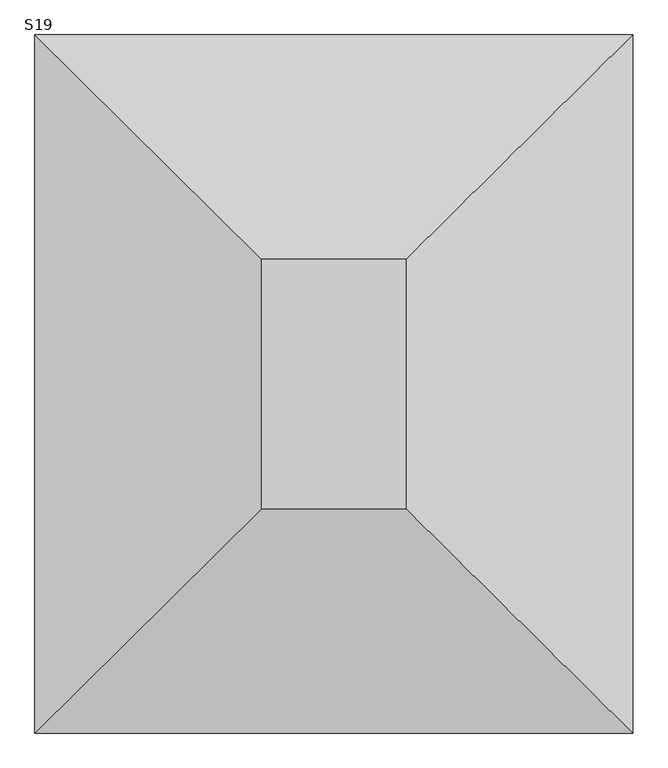
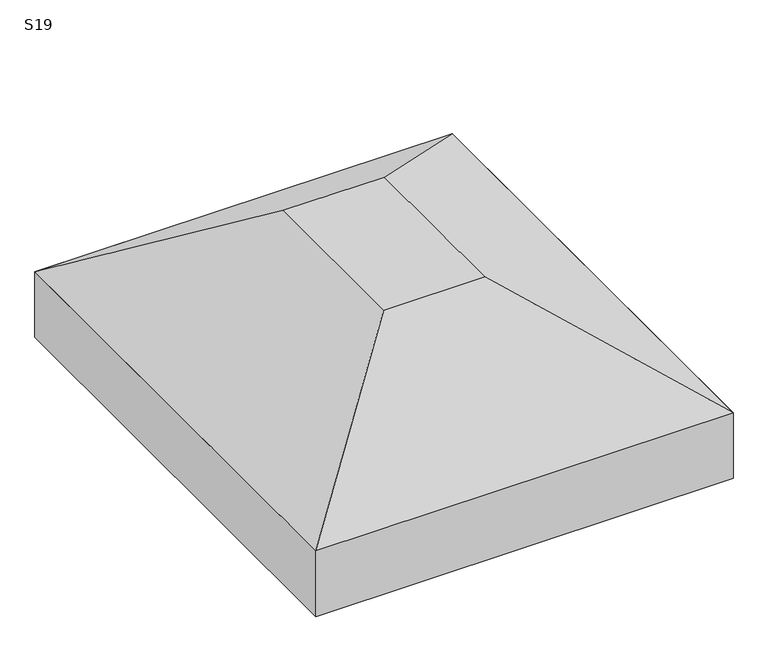
"""IFC4 building model written with IfcOpenShell, lengths in millimetres: fastener geometry, TQS - Sapata : S19."""

import ifcopenshell
import ifcopenshell.guid

model = None  # the IFC model being written
_history = None  # IfcOwnerHistory: only IFC2X3 demands one
_inside = {}  # id of a spatial element -> (the spatial element, [elements in it])
_under = {}  # id of a project, library or spatial element -> (it, [spatial elements below it])
_declared = {}  # id of a project -> (the project, [libraries it declares])
_typed = {}  # id of a type object -> (the type object, [elements of that type])
_made_of = {}  # id of a material, layer set ... -> (it, [elements and type objects made of it])


def new_model(schema):
    """Start an empty IFC model of exactly this schema.

    Asked for "IFC4X3", IfcOpenShell would pick the latest addendum, in which some entities
    have other attributes; the version numbers below select the first issue.
    IFC2X3 requires an IfcOwnerHistory on every rooted entity: one is made here for all.
    """
    global model, _history
    if schema == "IFC4X3":
        model = ifcopenshell.file(schema_version=(4, 3, 0, 0))
    else:
        model = ifcopenshell.file(schema=schema)
    _inside.clear()
    _under.clear()
    _declared.clear()
    _typed.clear()
    _made_of.clear()
    _history = None
    if model.schema == "IFC2X3":
        org = make("IfcOrganization", Name="unknown")
        user = make(
            "IfcPersonAndOrganization",
            ThePerson=make("IfcPerson", FamilyName="unknown"),
            TheOrganization=org,
        )
        app = make(
            "IfcApplication",
            ApplicationDeveloper=org,
            Version="unknown",
            ApplicationFullName="unknown",
            ApplicationIdentifier="unknown",
        )
        _history = make(
            "IfcOwnerHistory",
            OwningUser=user,
            OwningApplication=app,
            ChangeAction="ADDED",
            CreationDate=0,
        )
    return model


def make(cls, **values):
    """One entity of the class cls with the attributes given. An attribute that is None is left unset."""
    return model.create_entity(
        cls, **{name: value for name, value in values.items() if value is not None}
    )


def rooted(cls, **values):
    """An entity with a GlobalId (a new one), such as an element, a storey or a relation."""
    return make(cls, GlobalId=ifcopenshell.guid.new(), OwnerHistory=_history, **values)


def si_unit(unit_type, name, prefix=None):
    """IfcSIUnit, for example si_unit("LENGTHUNIT", "METRE", prefix="MILLI")."""
    return make("IfcSIUnit", UnitType=unit_type, Prefix=prefix, Name=name)


def assignment(units):
    """IfcUnitAssignment: the units of a project."""
    return None if units is None else make("IfcUnitAssignment", Units=units)


def point(xyz):
    """IfcCartesianPoint."""
    return None if xyz is None else make("IfcCartesianPoint", Coordinates=xyz)


def direction(xyz):
    """IfcDirection."""
    return None if xyz is None else make("IfcDirection", DirectionRatios=xyz)


def frame(location, z_axis=None, x_axis=None):
    """IfcAxis2Placement3D, a coordinate frame: its origin and axes. An axis left out is left unset."""
    return make(
        "IfcAxis2Placement3D",
        Location=point(location),
        Axis=direction(z_axis),
        RefDirection=direction(x_axis),
    )


def origin():
    """The frame at (0, 0, 0) with its axes left unset."""
    return frame((0.0, 0.0, 0.0))


def place(relative_to, where):
    """IfcLocalPlacement: puts the frame where relative to a parent placement (None: the world)."""
    return make(
        "IfcLocalPlacement", PlacementRelTo=relative_to, RelativePlacement=where
    )


def context(
    kind, dimensions, precision=None, world=None, true_north=None, identifier=None
):
    """IfcGeometricRepresentationContext, for example the 3D "Model" context."""
    return make(
        "IfcGeometricRepresentationContext",
        ContextIdentifier=identifier,
        ContextType=kind,
        CoordinateSpaceDimension=dimensions,
        Precision=precision,
        WorldCoordinateSystem=world,
        TrueNorth=true_north,
    )


def project(units=None, contexts=None):
    """IfcProject with its units and contexts."""
    return rooted(
        "IfcProject",
        Name="project",
        RepresentationContexts=contexts,
        UnitsInContext=assignment(units),
    )


def spatial(cls, under=None, at=None, **own):
    """A site, building, storey or space (cls), placed at a placement, below another one or the project."""
    s = rooted(cls, ObjectPlacement=at, **own)
    if under is not None:
        _under.setdefault(under.id(), (under, []))[1].append(s)
    return s


def polyline(points):
    """IfcPolyline through the points."""
    return make("IfcPolyline", Points=[point(p) for p in points])


def outline(outer, holes=None, kind="AREA"):
    """IfcArbitraryClosedProfileDef: a profile drawn as a closed curve; with holes, ...WithVoids."""
    if holes is None:
        return make("IfcArbitraryClosedProfileDef", ProfileType=kind, OuterCurve=outer)
    return make(
        "IfcArbitraryProfileDefWithVoids",
        ProfileType=kind,
        OuterCurve=outer,
        InnerCurves=holes,
    )


def extrude(swept, where, along, depth):
    """IfcExtrudedAreaSolid: the profile swept, set in the frame where, extruded along a direction by depth."""
    return make(
        "IfcExtrudedAreaSolid",
        SweptArea=swept,
        Position=where,
        ExtrudedDirection=direction(along),
        Depth=depth,
    )


def faces_of(points, faces, orient=None, outer=None):
    """IfcFace entities. A face is a list of loops; a loop is a list of indices into points, from 0.

    orient and outer hold one flag for each loop. By default every Orientation is true, the
    first loop of a face is its IfcFaceOuterBound and the others are IfcFaceBound.
    """
    made = []
    for i, loops in enumerate(faces):
        bounds = []
        for j, loop in enumerate(loops):
            is_outer = j == 0 if outer is None else outer[i][j]
            bounds.append(
                make(
                    "IfcFaceOuterBound" if is_outer else "IfcFaceBound",
                    Bound=make("IfcPolyLoop", Polygon=[points[k] for k in loop]),
                    Orientation=True if orient is None else orient[i][j],
                )
            )
        made.append(make("IfcFace", Bounds=bounds))
    return made


def faceted_brep(points, faces, orient=None, outer=None, voids=None):
    """IfcFacetedBrep: a solid bounded by flat faces; with voids (closed shells), ...WithVoids."""
    shared = [point(p) for p in points]
    hull = make("IfcClosedShell", CfsFaces=faces_of(shared, faces, orient, outer))
    if voids is None:
        return make("IfcFacetedBrep", Outer=hull)
    return make(
        "IfcFacetedBrepWithVoids",
        Outer=hull,
        Voids=[
            make(cls, CfsFaces=faces_of(shared, fs, o, b)) for cls, fs, o, b in voids
        ],
    )


def shape(context_of_items, identifier, shape_type, items):
    """IfcShapeRepresentation: the items that make up one representation, for example the "Body"."""
    return make(
        "IfcShapeRepresentation",
        ContextOfItems=context_of_items,
        RepresentationIdentifier=identifier,
        RepresentationType=shape_type,
        Items=items,
    )


def source(mapping_origin, context_of_items, identifier, shape_type, items):
    """IfcRepresentationMap: a shape defined once, which mapped items show again and again."""
    return make(
        "IfcRepresentationMap",
        MappingOrigin=mapping_origin,
        MappedRepresentation=shape(context_of_items, identifier, shape_type, items),
    )


def transform(
    local_origin,
    x_axis=None,
    y_axis=None,
    z_axis=None,
    scale=None,
    scale2=None,
    scale3=None,
    uniform=True,
):
    """IfcCartesianTransformationOperator3D, or its non-uniform kind. x_axis, y_axis, z_axis: its Axis1, 2, 3."""
    if uniform:
        return make(
            "IfcCartesianTransformationOperator3D",
            Axis1=direction(x_axis),
            Axis2=direction(y_axis),
            LocalOrigin=point(local_origin),
            Scale=scale,
            Axis3=direction(z_axis),
        )
    return make(
        "IfcCartesianTransformationOperator3DnonUniform",
        Axis1=direction(x_axis),
        Axis2=direction(y_axis),
        LocalOrigin=point(local_origin),
        Scale=scale,
        Axis3=direction(z_axis),
        Scale2=scale2,
        Scale3=scale3,
    )


def mapped(mapping_source, mapping_target):
    """IfcMappedItem: shows the shape of a source again, moved by a transform."""
    return make(
        "IfcMappedItem", MappingSource=mapping_source, MappingTarget=mapping_target
    )


def made_of(thing, what):
    """Note that an element or type object is made of a material, layer set ...; save() writes the relation."""
    if what is not None:
        _made_of.setdefault(what.id(), (what, []))[1].append(thing)
    return thing


def element(
    cls,
    number,
    at=None,
    inside=None,
    cuts=None,
    type_object=None,
    material=None,
    context=None,
    identifier="Body",
    shape_type=None,
    held_by="IfcProductDefinitionShape",
    body=None,
    shapes=None,
    **own,
):
    """One element of the class cls, such as IfcWall. Its Tag is "e" and its number.

    at: its placement. inside: the storey or other place that contains it. cuts: it is an
    opening in that element (IfcRelVoidsElement). A single representation is given by context,
    identifier, shape_type and body (its items); several are given by shapes. held_by: the class
    of the entity that holds the representations. save() writes the other relations.
    """
    e = rooted(cls, Tag="e%d" % number, ObjectPlacement=at, **own)
    if body is not None:
        shapes = [shape(context, identifier, shape_type, body)]
    if shapes is not None:
        e.Representation = make(held_by, Representations=shapes)
    if inside is not None:
        _inside.setdefault(inside.id(), (inside, []))[1].append(e)
    if cuts is not None:
        rooted(
            "IfcRelVoidsElement", RelatingBuildingElement=cuts, RelatedOpeningElement=e
        )
    if type_object is not None:
        _typed.setdefault(type_object.id(), (type_object, []))[1].append(e)
    return made_of(e, material)


def aggregate(whole, parts):
    """IfcRelAggregates: a whole, such as a stair, and the parts it consists of."""
    return rooted("IfcRelAggregates", RelatingObject=whole, RelatedObjects=parts)


def save(model, path):
    """Write the relations noted so far, then the file.

    IfcRelAggregates (storeys below a building ...), IfcRelContainedInSpatialStructure (elements
    in a storey), IfcRelDefinesByType, IfcRelAssociatesMaterial and IfcRelDeclares: one each for
    every whole, place, type object, material and project.
    """
    for whole, parts in _under.values():
        aggregate(whole, parts)
    for where, things in _inside.values():
        rooted(
            "IfcRelContainedInSpatialStructure",
            RelatedElements=things,
            RelatingStructure=where,
        )
    for kind, things in _typed.values():
        rooted("IfcRelDefinesByType", RelatedObjects=things, RelatingType=kind)
    for what, things in _made_of.values():
        rooted("IfcRelAssociatesMaterial", RelatedObjects=things, RelatingMaterial=what)
    for by, libraries in _declared.values():
        rooted("IfcRelDeclares", RelatingContext=by, RelatedDefinitions=libraries)
    model.write(path)


def s19_c62a4a8b(model_context):
    return source(origin(), model_context, "Body", "SolidModel", [
        faceted_brep([(-55.0, 50.0, 0.0), (-345.0, 50.0, 0.0), (-345.0, -450.0, 0.0), (-55.0, -450.0, 0.0), (400.0, 500.0, -300.0), (400.0, -900.0, -300.0), (-800.0, -900.0, -300.0), (-800.0, 500.0, -300.0)], [[[0, 1, 2, 3]], [[4, 5, 6, 7]], [[4, 7, 1, 0]], [[7, 6, 2, 1]], [[6, 5, 3, 2]], [[5, 4, 0, 3]]]),
        extrude(outline(polyline([(400.0, 500.0), (400.0, -900.0), (-800.0, -900.0), (-800.0, 500.0), (400.0, 500.0)])), frame((0.0, 0.0, -500.0), z_axis=(0.0, 0.0, 1.0), x_axis=(1.0, 0.0, 0.0)), (0.0, 0.0, 1.0), 200.0),
    ])


if __name__ == "__main__":
    model = new_model("IFC4")
    model_context = context("Model", 3, world=origin())
    ifc_project = project(units=[si_unit("LENGTHUNIT", "METRE", prefix="MILLI")], contexts=[model_context])
    site = spatial("IfcSite", under=ifc_project)
    building = spatial("IfcBuilding", under=site)
    placement = place(None, origin())
    s19_shape = s19_c62a4a8b(model_context)
    element("IfcFastener", 1, ObjectType="TQS - Sapata : S19", at=placement, inside=building, context=model_context, shape_type="MappedRepresentation", body=[
        mapped(s19_shape, transform((0.0, 0.0, 0.0), x_axis=(1.0, 0.0, 0.0), y_axis=(0.0, 1.0, 0.0), z_axis=(0.0, 0.0, 1.0))),
    ])
    save(model, "model.ifc")

# Revit data of these elements
# Type "TQS - Sapata : S19"
#   TY = 0.50 m
#   TX = 0.29 m
#   HS = 0.50 m
#   H0 = 0.20 m
#   EXCYABS = 0.70 m
#   EXCY = 0.00 m
#   EXCXABS = 0.60 m
#   EXCX = 0.00 m
#   DIMY = 1.40 m
#   DIMX = 1.20 m
#   Material estrutural = Concreto - Concreto concretado no local
#   Width = 0
#   Length = 0
# Element 1 (IfcFastener, "TQS - Sapata : S19")
#   Materials on its faces: "Concreto - Concreto concretado no local"
# Materials
#   "Concreto - Concreto concretado no local": class "Concreto", colour RGB 192 192 192, transparency 0
